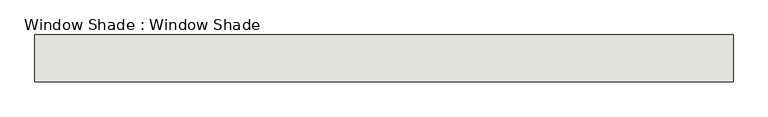
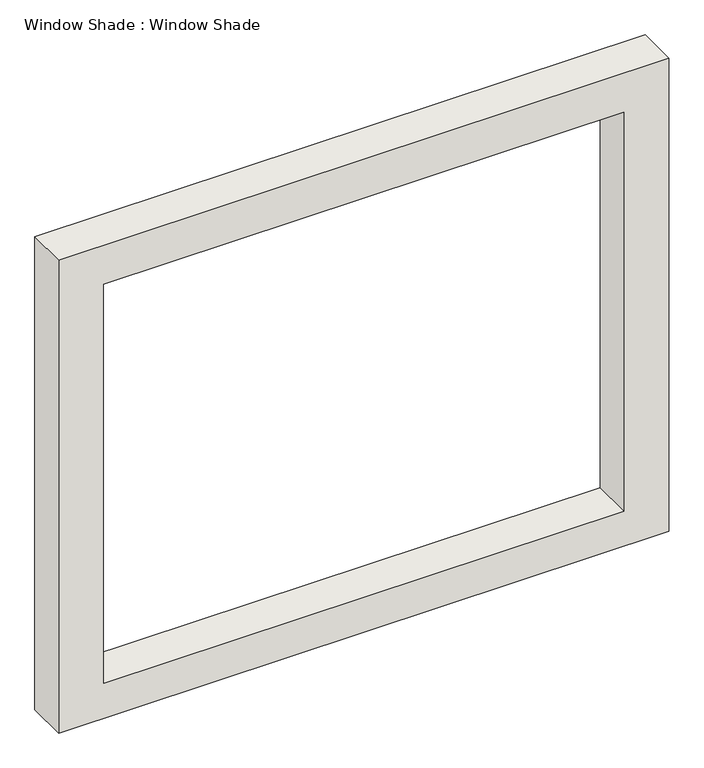
"""IFC4 building model written with IfcOpenShell, lengths in millimetres: wall geometry, Window Shade : Window Shade."""

import ifcopenshell
import ifcopenshell.guid

model = None  # the IFC model being written
_history = None  # IfcOwnerHistory: only IFC2X3 demands one
_inside = {}  # id of a spatial element -> (the spatial element, [elements in it])
_under = {}  # id of a project, library or spatial element -> (it, [spatial elements below it])
_declared = {}  # id of a project -> (the project, [libraries it declares])
_typed = {}  # id of a type object -> (the type object, [elements of that type])
_made_of = {}  # id of a material, layer set ... -> (it, [elements and type objects made of it])


def new_model(schema):
    """Start an empty IFC model of exactly this schema.

    Asked for "IFC4X3", IfcOpenShell would pick the latest addendum, in which some entities
    have other attributes; the version numbers below select the first issue.
    IFC2X3 requires an IfcOwnerHistory on every rooted entity: one is made here for all.
    """
    global model, _history
    if schema == "IFC4X3":
        model = ifcopenshell.file(schema_version=(4, 3, 0, 0))
    else:
        model = ifcopenshell.file(schema=schema)
    _inside.clear()
    _under.clear()
    _declared.clear()
    _typed.clear()
    _made_of.clear()
    _history = None
    if model.schema == "IFC2X3":
        org = make("IfcOrganization", Name="unknown")
        user = make(
            "IfcPersonAndOrganization",
            ThePerson=make("IfcPerson", FamilyName="unknown"),
            TheOrganization=org,
        )
        app = make(
            "IfcApplication",
            ApplicationDeveloper=org,
            Version="unknown",
            ApplicationFullName="unknown",
            ApplicationIdentifier="unknown",
        )
        _history = make(
            "IfcOwnerHistory",
            OwningUser=user,
            OwningApplication=app,
            ChangeAction="ADDED",
            CreationDate=0,
        )
    return model


def make(cls, **values):
    """One entity of the class cls with the attributes given. An attribute that is None is left unset."""
    return model.create_entity(
        cls, **{name: value for name, value in values.items() if value is not None}
    )


def rooted(cls, **values):
    """An entity with a GlobalId (a new one), such as an element, a storey or a relation."""
    return make(cls, GlobalId=ifcopenshell.guid.new(), OwnerHistory=_history, **values)


def si_unit(unit_type, name, prefix=None):
    """IfcSIUnit, for example si_unit("LENGTHUNIT", "METRE", prefix="MILLI")."""
    return make("IfcSIUnit", UnitType=unit_type, Prefix=prefix, Name=name)


def assignment(units):
    """IfcUnitAssignment: the units of a project."""
    return None if units is None else make("IfcUnitAssignment", Units=units)


def point(xyz):
    """IfcCartesianPoint."""
    return None if xyz is None else make("IfcCartesianPoint", Coordinates=xyz)


def direction(xyz):
    """IfcDirection."""
    return None if xyz is None else make("IfcDirection", DirectionRatios=xyz)


def frame(location, z_axis=None, x_axis=None):
    """IfcAxis2Placement3D, a coordinate frame: its origin and axes. An axis left out is left unset."""
    return make(
        "IfcAxis2Placement3D",
        Location=point(location),
        Axis=direction(z_axis),
        RefDirection=direction(x_axis),
    )


def origin():
    """The frame at (0, 0, 0) with its axes left unset."""
    return frame((0.0, 0.0, 0.0))


def place(relative_to, where):
    """IfcLocalPlacement: puts the frame where relative to a parent placement (None: the world)."""
    return make(
        "IfcLocalPlacement", PlacementRelTo=relative_to, RelativePlacement=where
    )


def context(
    kind, dimensions, precision=None, world=None, true_north=None, identifier=None
):
    """IfcGeometricRepresentationContext, for example the 3D "Model" context."""
    return make(
        "IfcGeometricRepresentationContext",
        ContextIdentifier=identifier,
        ContextType=kind,
        CoordinateSpaceDimension=dimensions,
        Precision=precision,
        WorldCoordinateSystem=world,
        TrueNorth=true_north,
    )


def project(units=None, contexts=None):
    """IfcProject with its units and contexts."""
    return rooted(
        "IfcProject",
        Name="project",
        RepresentationContexts=contexts,
        UnitsInContext=assignment(units),
    )


def spatial(cls, under=None, at=None, **own):
    """A site, building, storey or space (cls), placed at a placement, below another one or the project."""
    s = rooted(cls, ObjectPlacement=at, **own)
    if under is not None:
        _under.setdefault(under.id(), (under, []))[1].append(s)
    return s


def polyline(points):
    """IfcPolyline through the points."""
    return make("IfcPolyline", Points=[point(p) for p in points])


def outline(outer, holes=None, kind="AREA"):
    """IfcArbitraryClosedProfileDef: a profile drawn as a closed curve; with holes, ...WithVoids."""
    if holes is None:
        return make("IfcArbitraryClosedProfileDef", ProfileType=kind, OuterCurve=outer)
    return make(
        "IfcArbitraryProfileDefWithVoids",
        ProfileType=kind,
        OuterCurve=outer,
        InnerCurves=holes,
    )


def extrude(swept, where, along, depth):
    """IfcExtrudedAreaSolid: the profile swept, set in the frame where, extruded along a direction by depth."""
    return make(
        "IfcExtrudedAreaSolid",
        SweptArea=swept,
        Position=where,
        ExtrudedDirection=direction(along),
        Depth=depth,
    )


def shape(context_of_items, identifier, shape_type, items):
    """IfcShapeRepresentation: the items that make up one representation, for example the "Body"."""
    return make(
        "IfcShapeRepresentation",
        ContextOfItems=context_of_items,
        RepresentationIdentifier=identifier,
        RepresentationType=shape_type,
        Items=items,
    )


def source(mapping_origin, context_of_items, identifier, shape_type, items):
    """IfcRepresentationMap: a shape defined once, which mapped items show again and again."""
    return make(
        "IfcRepresentationMap",
        MappingOrigin=mapping_origin,
        MappedRepresentation=shape(context_of_items, identifier, shape_type, items),
    )


def transform(
    local_origin,
    x_axis=None,
    y_axis=None,
    z_axis=None,
    scale=None,
    scale2=None,
    scale3=None,
    uniform=True,
):
    """IfcCartesianTransformationOperator3D, or its non-uniform kind. x_axis, y_axis, z_axis: its Axis1, 2, 3."""
    if uniform:
        return make(
            "IfcCartesianTransformationOperator3D",
            Axis1=direction(x_axis),
            Axis2=direction(y_axis),
            LocalOrigin=point(local_origin),
            Scale=scale,
            Axis3=direction(z_axis),
        )
    return make(
        "IfcCartesianTransformationOperator3DnonUniform",
        Axis1=direction(x_axis),
        Axis2=direction(y_axis),
        LocalOrigin=point(local_origin),
        Scale=scale,
        Axis3=direction(z_axis),
        Scale2=scale2,
        Scale3=scale3,
    )


def mapped(mapping_source, mapping_target):
    """IfcMappedItem: shows the shape of a source again, moved by a transform."""
    return make(
        "IfcMappedItem", MappingSource=mapping_source, MappingTarget=mapping_target
    )


def made_of(thing, what):
    """Note that an element or type object is made of a material, layer set ...; save() writes the relation."""
    if what is not None:
        _made_of.setdefault(what.id(), (what, []))[1].append(thing)
    return thing


def element(
    cls,
    number,
    at=None,
    inside=None,
    cuts=None,
    type_object=None,
    material=None,
    context=None,
    identifier="Body",
    shape_type=None,
    held_by="IfcProductDefinitionShape",
    body=None,
    shapes=None,
    **own,
):
    """One element of the class cls, such as IfcWall. Its Tag is "e" and its number.

    at: its placement. inside: the storey or other place that contains it. cuts: it is an
    opening in that element (IfcRelVoidsElement). A single representation is given by context,
    identifier, shape_type and body (its items); several are given by shapes. held_by: the class
    of the entity that holds the representations. save() writes the other relations.
    """
    e = rooted(cls, Tag="e%d" % number, ObjectPlacement=at, **own)
    if body is not None:
        shapes = [shape(context, identifier, shape_type, body)]
    if shapes is not None:
        e.Representation = make(held_by, Representations=shapes)
    if inside is not None:
        _inside.setdefault(inside.id(), (inside, []))[1].append(e)
    if cuts is not None:
        rooted(
            "IfcRelVoidsElement", RelatingBuildingElement=cuts, RelatedOpeningElement=e
        )
    if type_object is not None:
        _typed.setdefault(type_object.id(), (type_object, []))[1].append(e)
    return made_of(e, material)


def aggregate(whole, parts):
    """IfcRelAggregates: a whole, such as a stair, and the parts it consists of."""
    return rooted("IfcRelAggregates", RelatingObject=whole, RelatedObjects=parts)


def save(model, path):
    """Write the relations noted so far, then the file.

    IfcRelAggregates (storeys below a building ...), IfcRelContainedInSpatialStructure (elements
    in a storey), IfcRelDefinesByType, IfcRelAssociatesMaterial and IfcRelDeclares: one each for
    every whole, place, type object, material and project.
    """
    for whole, parts in _under.values():
        aggregate(whole, parts)
    for where, things in _inside.values():
        rooted(
            "IfcRelContainedInSpatialStructure",
            RelatedElements=things,
            RelatingStructure=where,
        )
    for kind, things in _typed.values():
        rooted("IfcRelDefinesByType", RelatedObjects=things, RelatingType=kind)
    for what, things in _made_of.values():
        rooted("IfcRelAssociatesMaterial", RelatedObjects=things, RelatingMaterial=what)
    for by, libraries in _declared.values():
        rooted("IfcRelDeclares", RelatingContext=by, RelatedDefinitions=libraries)
    model.write(path)


def window_shade_window_shade_60a7ed7f(model_context):
    return source(origin(), model_context, "Body", "SweptSolid", [
        extrude(outline(polyline([(2152.65, 8426.2909002), (2152.65, 6533.9909002), (603.25, 6533.9909002), (603.25, 8426.2909002), (2152.65, 8426.2909002)]), holes=[polyline([(2025.65, 8286.5909002), (717.55, 8286.5909002), (717.55, 6673.6909002), (2025.65, 6673.6909002), (2025.65, 8286.5909002)])]), frame((0.0, -15471.0114294, 0.0), z_axis=(0.0, 1.0, 0.0), x_axis=(0.0, 0.0, 1.0)), (0.0, 0.0, 1.0), 127.0),
    ])


if __name__ == "__main__":
    model = new_model("IFC4")
    model_context = context("Model", 3, world=origin())
    ifc_project = project(units=[si_unit("LENGTHUNIT", "METRE", prefix="MILLI")], contexts=[model_context])
    site = spatial("IfcSite", under=ifc_project)
    building = spatial("IfcBuilding", under=site)
    placement = place(None, origin())
    window_shade_window_shade_shape = window_shade_window_shade_60a7ed7f(model_context)
    element("IfcWall", 1, ObjectType="Window Shade : Window Shade", at=placement, inside=building, context=model_context, shape_type="MappedRepresentation", body=[
        mapped(window_shade_window_shade_shape, transform((0.0, 0.0, 0.0), x_axis=(1.0, 0.0, 0.0), y_axis=(0.0, 1.0, 0.0), z_axis=(0.0, 0.0, 1.0))),
    ])
    save(model, "model.ifc")

# Revit data of these elements
# Element 1 (IfcWall, "Window Shade : Window Shade")
#   Materials on its faces: "Wood Planks"
# Materials
#   "Wood Planks": class "Wood", colour RGB 129 72 39, transparency 0, Description = "Physical material.", Cost = 0
